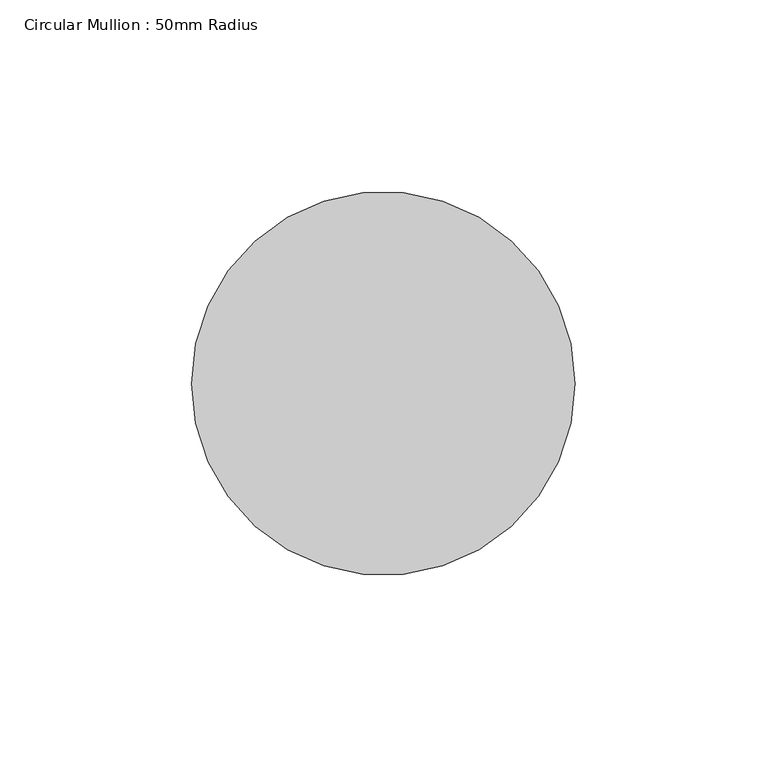
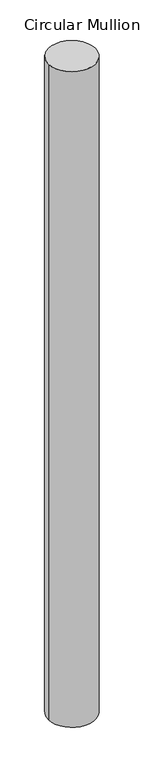
"""IFC4 building model written with IfcOpenShell, lengths in millimetres: member geometry, Circular Mullion : 50mm Radius."""

from ifc_helpers import new_model, si_unit, point, frame, origin, origin_2d, place, context, project, spatial, circle_curve, trimmed, segment, composite_curve, outline, extrude, source, transform, mapped, element, save


def circular_mullion_50mm_radius_e463ac65(model_context):
    return source(origin(), model_context, "Body", "SweptSolid", [
        extrude(outline(composite_curve([segment(trimmed(circle_curve(origin_2d(), 50.0), [point((50.0, 0.0))], [point((-50.0, 0.0))], False, "CARTESIAN"), True, "CONTINUOUS"), segment(trimmed(circle_curve(origin_2d(), 50.0), [point((-50.0, 0.0))], [point((50.0, 0.0))], False, "CARTESIAN"), True, "CONTINUOUS")], self_intersect=False)), frame((0.0, 0.0, -1471.9925615), z_axis=(0.0, 0.0, 1.0), x_axis=(1.0, 0.0, 0.0)), (0.0, 0.0, 1.0), 1471.9925615),
    ])


if __name__ == "__main__":
    model = new_model("IFC4")
    model_context = context("Model", 3, world=origin())
    ifc_project = project(units=[si_unit("LENGTHUNIT", "METRE", prefix="MILLI")], contexts=[model_context])
    site = spatial("IfcSite", under=ifc_project)
    building = spatial("IfcBuilding", under=site)
    placement = place(None, origin())
    circular_mullion_50mm_radius_shape = circular_mullion_50mm_radius_e463ac65(model_context)
    element("IfcMember", 1, ObjectType="Circular Mullion : 50mm Radius", at=placement, inside=building, context=model_context, shape_type="MappedRepresentation", body=[
        mapped(circular_mullion_50mm_radius_shape, transform((0.0, 0.0, 0.0), x_axis=(1.0, 0.0, 0.0), y_axis=(0.0, 1.0, 0.0), z_axis=(0.0, 0.0, 1.0))),
    ])
    save(model, "model.ifc")

# Revit data of these elements
# Type "Circular Mullion : 50mm Radius"
#   built-in parameter 1007350 = 0.164042 (stored number, unit not read)
# Element 1 (IfcMember, "Circular Mullion : 50mm Radius")
#   Materials on its faces: "Aluminium"
# Materials
#   "Aluminium": class "Metal", colour RGB 247 247 247, transparency 0, Description = "Aluminium 6061", Cost = 0
